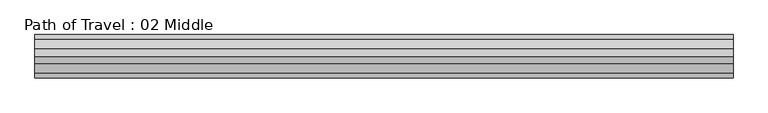
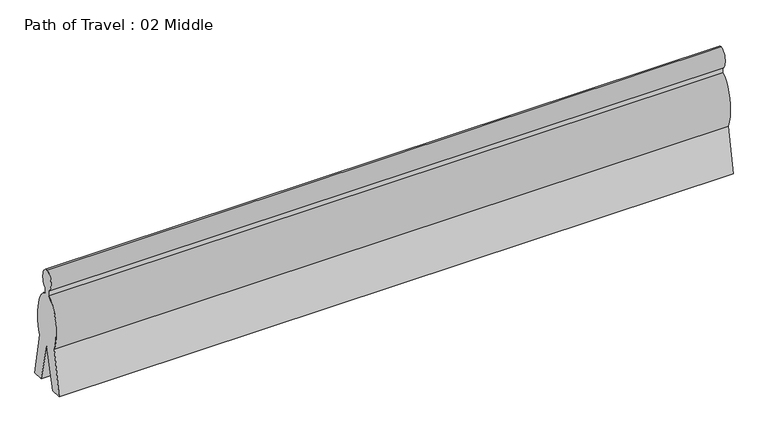
"""IFC4 building model written with IfcOpenShell, lengths in millimetres: proxy geometry, Path of Travel : 02 Middle."""

from ifc_helpers import new_model, si_unit, point, frame, origin, place, context, project, spatial, ellipse_curve, trimmed, source, transform, mapped, element, save
from ifc_brep_helpers import plane_surface, extruded_surface, advanced_brep


def path_of_travel_02_middle_0399148d(model_context):
    return source(origin(), model_context, "Body", "AdvancedBrep", [
        advanced_brep(
        [(227.5554837, 0.0, 1727.2), (227.5554837, 42.9018657, 1436.6534209), (227.5554837, 42.9018657, 1363.4763406), (227.5554837, 184.1186263, 643.4144547), (227.5554837, 297.5699544, 0.0), (227.5554837, 145.6574193, 0.0), (227.5554837, 0.0, 584.2), (227.5554837, -145.6574193, 0.0), (227.5554837, -297.5699544, 0.0), (227.5554837, -184.1186263, 643.4144547), (227.5554837, -42.9018657, 1363.4763406), (227.5554837, -42.9018657, 1436.6534209), (9828.7554837, 0.0, 1727.2), (9828.7554837, -42.9018657, 1436.6534209), (9828.7554837, -42.9018657, 1363.4763406), (9828.7554837, -184.1186263, 643.4144547), (9828.7554837, -297.5699544, 0.0), (9828.7554837, -145.6574193, 0.0), (9828.7554837, 0.0, 584.2), (9828.7554837, 145.6574193, 0.0), (9828.7554837, 297.5699544, 0.0), (9828.7554837, 184.1186263, 643.4144547), (9828.7554837, 42.9018657, 1363.4763406), (9828.7554837, 42.9018657, 1436.6534209)],
        [
            (0, 1, ellipse_curve(frame((227.5554837, 0.0, 1574.8), z_axis=(-1.0, 0.0, 0.0), x_axis=(0.0, 0.0, 1.0)), 152.4, 101.6)),
            (1, 2),
            (2, 3, ellipse_curve(frame((227.5554837, 0.0, 914.4), z_axis=(-1.0, 0.0, 0.0), x_axis=(0.0, 0.0, -1.0)), 457.2, 228.6)),
            (3, 4),
            (4, 5),
            (5, 6),
            (6, 7),
            (7, 8),
            (8, 9),
            (9, 10, ellipse_curve(frame((227.5554837, 0.0, 914.4), z_axis=(-1.0, 0.0, 0.0), x_axis=(0.0, 0.0, -1.0)), 457.2, 228.6)),
            (10, 11),
            (11, 0, ellipse_curve(frame((227.5554837, 0.0, 1574.8), z_axis=(-1.0, 0.0, 0.0), x_axis=(0.0, 0.0, 1.0)), 152.4, 101.6)),
            (12, 13, ellipse_curve(frame((9828.7554837, 0.0, 1574.8), z_axis=(1.0, 0.0, 0.0), x_axis=(0.0, 0.0, 1.0)), 152.4, 101.6)),
            (13, 14),
            (14, 15, ellipse_curve(frame((9828.7554837, 0.0, 914.4), z_axis=(1.0, 0.0, 0.0), x_axis=(0.0, 0.0, -1.0)), 457.2, 228.6)),
            (15, 16),
            (16, 17),
            (17, 18),
            (18, 19),
            (19, 20),
            (20, 21),
            (21, 22, ellipse_curve(frame((9828.7554837, 0.0, 914.4), z_axis=(1.0, 0.0, 0.0), x_axis=(0.0, 0.0, -1.0)), 457.2, 228.6)),
            (22, 23),
            (23, 12, ellipse_curve(frame((9828.7554837, 0.0, 1574.8), z_axis=(1.0, 0.0, 0.0), x_axis=(0.0, 0.0, 1.0)), 152.4, 101.6)),
            (0, 12),
            (23, 1),
            (22, 2),
            (21, 3),
            (20, 4),
            (19, 5),
            (18, 6),
            (17, 7),
            (16, 8),
            (15, 9),
            (14, 10),
            (13, 11),
        ],
        [
            plane_surface(frame((227.5554837, 0.0, 0.0), z_axis=(-1.0, 0.0, 0.0), x_axis=(0.0, 0.0, 1.0))),
            plane_surface(frame((9828.7554837, 0.0, 0.0), z_axis=(1.0, 0.0, 0.0), x_axis=(0.0, 0.0, 1.0))),
            extruded_surface(trimmed(ellipse_curve(frame((9828.7554837, 0.0, 1574.8), z_axis=(-1.0, 0.0, 0.0), x_axis=(0.0, 0.0, 1.0)), 152.4, 101.6), [point((9828.7554837, 0.0, 1727.2))], [point((9828.7554837, 42.9018657, 1436.6534209))], True, "CARTESIAN"), (-9601.2, 0.0, 0.0), 9601.2),
            plane_surface(frame((227.5554837, 42.9018657, 1436.6534209), z_axis=(0.0, 1.0, 0.0), x_axis=(1.0, 0.0, 0.0))),
            extruded_surface(trimmed(ellipse_curve(frame((9828.7554837, 0.0, 914.4), z_axis=(-1.0, 0.0, 0.0), x_axis=(0.0, 0.0, -1.0)), 457.2, 228.6), [point((9828.7554837, 42.9018657, 1363.4763406))], [point((9828.7554837, 184.1186263, 643.4144547))], True, "CARTESIAN"), (-9601.2, 0.0, 0.0), 9601.2),
            plane_surface(frame((227.5554837, 184.1186263, 643.4144547), z_axis=(0.0, 0.9848077530122078, 0.17364817766693205), x_axis=(1.0, 0.0, 0.0))),
            plane_surface(frame((227.5554837, 297.5699544, 0.0), z_axis=(0.0, 0.0, -1.0), x_axis=(1.0, 0.0, 0.0))),
            plane_surface(frame((227.5554837, 145.6574193, 0.0), z_axis=(0.0, -0.9702957262760199, -0.2419218955995739), x_axis=(1.0, 0.0, 0.0))),
            plane_surface(frame((227.5554837, 0.0, 584.2), z_axis=(0.0, 0.9702957262759961, -0.24192189559966923), x_axis=(1.0, 0.0, 0.0))),
            plane_surface(frame((227.5554837, -145.6574193, 0.0), z_axis=(0.0, 0.0, -1.0), x_axis=(1.0, 0.0, 0.0))),
            plane_surface(frame((227.5554837, -297.5699544, 0.0), z_axis=(0.0, -0.984807753012208, 0.17364817766693066), x_axis=(1.0, 0.0, 0.0))),
            extruded_surface(trimmed(ellipse_curve(frame((9828.7554837, 0.0, 914.4), z_axis=(-1.0, 0.0, 0.0), x_axis=(0.0, 0.0, -1.0)), 457.2, 228.6), [point((9828.7554837, -184.1186263, 643.4144547))], [point((9828.7554837, -42.9018657, 1363.4763406))], True, "CARTESIAN"), (-9601.2, 0.0, 0.0), 9601.2),
            plane_surface(frame((227.5554837, -42.9018657, 1363.4763406), z_axis=(0.0, -1.0, 0.0), x_axis=(1.0, 0.0, 0.0))),
            extruded_surface(trimmed(ellipse_curve(frame((9828.7554837, 0.0, 1574.8), z_axis=(-1.0, 0.0, 0.0), x_axis=(0.0, 0.0, 1.0)), 152.4, 101.6), [point((9828.7554837, -42.9018657, 1436.6534209))], [point((9828.7554837, 0.0, 1727.2))], True, "CARTESIAN"), (-9601.2, 0.0, 0.0), 9601.2),
        ],
        [
            (0, [[1, 2, 3, 4, 5, 6, 7, 8, 9, 10, 11, 12]]),
            (1, [[13, 14, 15, 16, 17, 18, 19, 20, 21, 22, 23, 24]]),
            (2, [[-1, 25, -24, 26]]),
            (3, [[-2, -26, -23, 27]]),
            (4, [[-3, -27, -22, 28]]),
            (5, [[-4, -28, -21, 29]]),
            (6, [[-5, -29, -20, 30]]),
            (7, [[-6, -30, -19, 31]]),
            (8, [[-7, -31, -18, 32]]),
            (9, [[-8, -32, -17, 33]]),
            (10, [[-9, -33, -16, 34]]),
            (11, [[-10, -34, -15, 35]]),
            (12, [[-11, -35, -14, 36]]),
            (13, [[-12, -36, -13, -25]]),
        ],
    ),
    ])


if __name__ == "__main__":
    model = new_model("IFC4")
    model_context = context("Model", 3, world=origin())
    ifc_project = project(units=[si_unit("LENGTHUNIT", "METRE", prefix="MILLI")], contexts=[model_context])
    site = spatial("IfcSite", under=ifc_project)
    building = spatial("IfcBuilding", under=site)
    placement = place(None, origin())
    path_of_travel_02_middle_shape = path_of_travel_02_middle_0399148d(model_context)
    element("IfcBuildingElementProxy", 1, Name="Path of Travel : 02 Middle", ObjectType="Path of Travel : 02 Middle", at=placement, inside=building, context=model_context, shape_type="MappedRepresentation", body=[
        mapped(path_of_travel_02_middle_shape, transform((0.0, 0.0, 0.0), x_axis=(1.0, 0.0, 0.0), y_axis=(0.0, 1.0, 0.0), z_axis=(0.0, 0.0, 1.0))),
    ])
    save(model, "model.ifc")

# Revit data of these elements
# Type "Path of Travel : 02 Middle"
#   Path of Egress [instance default] = 4' - 0"
#   built-in parameter 1001306 [instance default] = 4 (stored number, unit not read)
#   Dot at Start = no
#   Arrow in Middle = yes
#   Arrow at End = no
#   Egress Path = none
# Element 1 (IfcBuildingElementProxy, "Path of Travel : 02 Middle")
#   Path of Egress = 31' - 6"
#   built-in parameter 1001306 = 31.5 (stored number, unit not read)
#   Materials on its faces: "Egress Path Solid"
# Materials
#   "Egress Path Solid": class "Unassigned", colour RGB 255 128 64, transparency 0.75, Comments = "Rendering appearance not upgraded "
